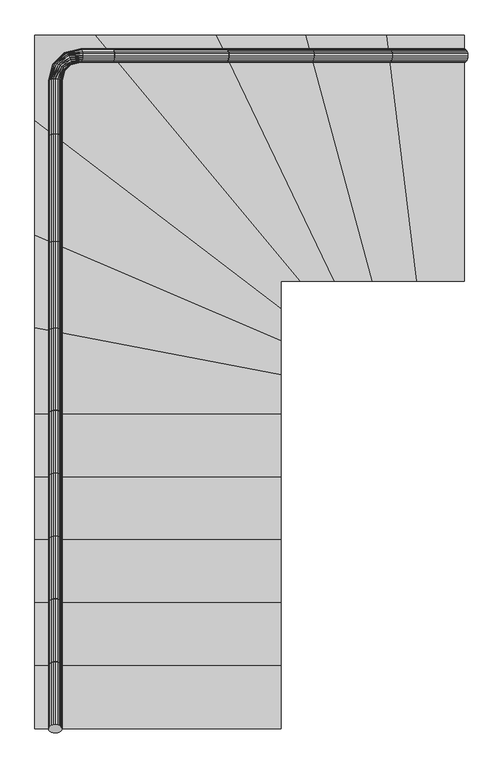
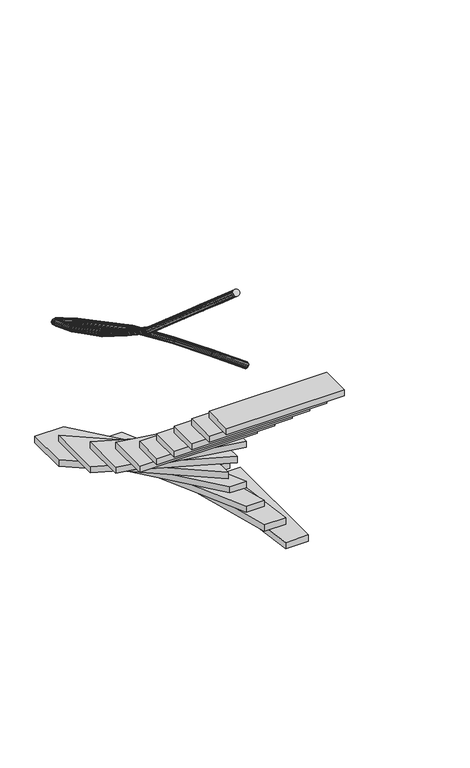
"""IFC4 building model written with IfcOpenShell, lengths in millimetres: stair geometry, 0_3d."""

from ifc_helpers import new_model, si_unit, frame, origin, origin_with_axes, place, context, project, spatial, polyline, outline, extrude, faceted_brep, source, transform, mapped, element, save


def stair_f0ca9b28(model_context):
    return source(origin(), model_context, "Body", "SolidModel", [
        extrude(outline(polyline([(1231.3290941, 1649.6053406), (1093.3486159, 1649.6053406), (662.4236343, 2549.6053406), (988.6709059, 2549.6053406), (1231.3290941, 1649.6053406)])), frame((0.0, 0.0, 400.0), z_axis=(0.0, 0.0, 1.0), x_axis=(1.0, 0.0, 0.0)), (0.0, 0.0, 1.0), 50.0),
        extrude(outline(polyline([(900.0, 705.003504), (900.0, 475.003504), (0.0, 475.003504), (0.0, 705.003504), (900.0, 705.003504)])), frame((0.0, 0.0, 2000.0), z_axis=(0.0, 0.0, 1.0), x_axis=(1.0, 0.0, 0.0)), (0.0, 0.0, 1.0), 50.0),
        extrude(outline(polyline([(1093.3486159, 1649.6053406), (970.0, 1649.6053406), (219.7566439, 2549.6053406), (662.4236343, 2549.6053406), (1093.3486159, 1649.6053406)])), frame((0.0, 0.0, 600.0), z_axis=(0.0, 0.0, 1.0), x_axis=(1.0, 0.0, 0.0)), (0.0, 0.0, 1.0), 50.0),
        extrude(outline(polyline([(1.2235871, -7.0656631), (0.0, 0.0), (1.2235871, 7.0656631), (4.7745751, 13.4396897), (10.3053687, 18.4981459), (17.2745751, 21.7458748), (25.0, 22.8649659), (32.7254249, 21.7458748), (39.6946313, 18.4981459), (45.2254249, 13.4396897), (48.7764129, 7.0656631), (50.0, 0.0), (48.7764129, -7.0656631), (45.2254249, -13.4396898), (39.6946313, -18.498146), (32.7254249, -21.7458748), (25.0, -22.864966), (17.2745751, -21.7458748), (10.3053687, -18.498146), (4.7745751, -13.4396898), (1.2235871, -7.0656631)])), frame((50.0, 475.003504, 3121.0), z_axis=(0.0, -0.7546055221635335, 0.6561787149247537), x_axis=(1.0, 0.0, 0.0)), (0.0, 0.0, 1.0), 304.7950131),
        extrude(outline(polyline([(1570.0, 1649.6053406), (1394.8371648, 1649.6053406), (1285.1628352, 2549.6053406), (1570.0, 2549.6053406), (1570.0, 1649.6053406)])), origin_with_axes(), (0.0, 0.0, 1.0), 50.0),
        extrude(outline(polyline([(1.2235871, -7.0656631), (0.0, 0.0), (1.2235871, 7.0656631), (4.7745751, 13.4396897), (10.3053687, 18.4981459), (17.2745751, 21.7458748), (25.0, 22.8649659), (32.7254249, 21.7458748), (39.6946313, 18.4981459), (45.2254249, 13.4396897), (48.7764129, 7.0656631), (50.0, 0.0), (48.7764129, -7.0656631), (45.2254249, -13.4396898), (39.6946313, -18.498146), (32.7254249, -21.7458748), (25.0, -22.864966), (17.2745751, -21.7458748), (10.3053687, -18.498146), (4.7745751, -13.4396898), (1.2235871, -7.0656631)])), frame((50.0, 935.003504, 2721.0), z_axis=(0.0, -0.7546055221635325, 0.6561787149247547), x_axis=(1.0, 0.0, 0.0)), (0.0, 0.0, 1.0), 304.7950131),
        faceted_brep([(51.2235871, 2175.7019192, 1914.5547212), (50.0, 2178.6155291, 1921.0), (51.2235871, 2181.5291389, 1927.4452788), (54.7745751, 2184.1575443, 1933.2596488), (60.3053687, 2186.2434586, 1937.8739589), (67.2745751, 2187.5826981, 1940.8365284), (75.0, 2188.0441685, 1941.8573603), (82.7254249, 2187.5826981, 1940.8365284), (89.6946313, 2186.2434586, 1937.8739589), (95.2254249, 2184.1575443, 1933.2596488), (98.7764129, 2181.5291389, 1927.4452788), (100.0, 2178.6155291, 1921.0), (98.7764129, 2175.7019192, 1914.5547212), (95.2254249, 2173.0735138, 1908.7403512), (89.6946313, 2170.9875995, 1904.1260411), (82.7254249, 2169.64836, 1901.1634716), (75.0, 2169.1868896, 1900.1426397), (67.2745751, 2169.64836, 1901.1634716), (60.3053687, 2170.9875995, 1904.1260411), (54.7745751, 2173.0735138, 1908.7403512), (51.2235871, 1789.2064798, 2127.1536239), (50.0, 1785.7199202, 2121.0), (51.2235871, 1782.2333607, 2114.8463761), (54.7745751, 1779.0880899, 2109.2951119), (60.3053687, 1776.5919889, 2104.8896036), (67.2745751, 1774.9893933, 2102.0610932), (75.0, 1774.4371766, 2101.0864549), (82.7254249, 1774.9893933, 2102.0610932), (89.6946313, 1776.5919889, 2104.8896036), (95.2254249, 1779.0880899, 2109.2951119), (98.7764129, 1782.2333607, 2114.8463761), (100.0, 1785.7199202, 2121.0), (98.7764129, 1789.2064798, 2127.1536239), (95.2254249, 1792.3517506, 2132.7048881), (89.6946313, 1794.8478516, 2137.1103964), (82.7254249, 1796.4504471, 2139.9389068), (75.0, 1797.0026639, 2140.9135451), (67.2745751, 1796.4504471, 2139.9389068), (60.3053687, 1794.8478516, 2137.1103964), (54.7745751, 1792.3517506, 2132.7048881)], [[[0, 1, 2, 3, 4, 5, 6, 7, 8, 9, 10, 11, 12, 13, 14, 15, 16, 17, 18, 19]], [[20, 21, 22, 23, 24, 25, 26, 27, 28, 29, 30, 31, 32, 33, 34, 35, 36, 37, 38, 39]], [[2, 1, 21, 20]], [[3, 2, 20, 39]], [[4, 3, 39, 38]], [[5, 4, 38, 37]], [[6, 5, 37, 36]], [[7, 6, 36, 35]], [[8, 7, 35, 34]], [[9, 8, 34, 33]], [[10, 9, 33, 32]], [[11, 10, 32, 31]], [[12, 11, 31, 30]], [[13, 12, 30, 29]], [[14, 13, 29, 28]], [[15, 14, 28, 27]], [[16, 15, 27, 26]], [[17, 16, 26, 25]], [[18, 17, 25, 24]], [[19, 18, 24, 23]], [[0, 19, 23, 22]], [[1, 0, 22, 21]]]),
        extrude(outline(polyline([(1.2235871, -7.0656631), (0.0, 0.0), (1.2235871, 7.0656631), (4.7745751, 13.4396897), (10.3053687, 18.4981459), (17.2745751, 21.7458748), (25.0, 22.8649659), (32.7254249, 21.7458748), (39.6946313, 18.4981459), (45.2254249, 13.4396897), (48.7764129, 7.0656631), (50.0, 0.0), (48.7764129, -7.0656631), (45.2254249, -13.4396898), (39.6946313, -18.498146), (32.7254249, -21.7458748), (25.0, -22.864966), (17.2745751, -21.7458748), (10.3053687, -18.498146), (4.7745751, -13.4396898), (1.2235871, -7.0656631)])), frame((50.0, 245.003504, 3321.0), z_axis=(0.0, -0.7546055221635316, 0.6561787149247558), x_axis=(1.0, 0.0, 0.0)), (0.0, 0.0, 1.0), 304.7950131),
        extrude(outline(polyline([(1.2235871, -7.0656631), (0.0, 0.0), (1.2235871, 7.0656631), (4.7745751, 13.4396897), (10.3053687, 18.4981459), (17.2745751, 21.7458748), (25.0, 22.8649659), (32.7254249, 21.7458748), (39.6946313, 18.4981459), (45.2254249, 13.4396897), (48.7764129, 7.0656631), (50.0, 0.0), (48.7764129, -7.0656631), (45.2254249, -13.4396898), (39.6946313, -18.498146), (32.7254249, -21.7458748), (25.0, -22.864966), (17.2745751, -21.7458748), (10.3053687, -18.498146), (4.7745751, -13.4396898), (1.2235871, -7.0656631)])), frame((50.0, 705.003504, 2921.0), z_axis=(0.0, -0.7546055221635325, 0.6561787149247547), x_axis=(1.0, 0.0, 0.0)), (0.0, 0.0, 1.0), 304.7950131),
        faceted_brep([(1004.9507123, 2498.3817535, 1315.1343723), (1008.8924216, 2499.6053406, 1321.0), (1012.8341309, 2498.3817535, 1326.8656277), (1016.3899982, 2494.8307654, 1332.1570869), (1019.2119505, 2489.2999719, 1336.3564127), (1021.0237554, 2482.3307654, 1339.0525459), (1021.6480608, 2474.6053406, 1339.98157), (1021.0237554, 2466.8799157, 1339.0525459), (1019.2119505, 2459.9107093, 1336.3564127), (1016.3899982, 2454.3799157, 1332.1570869), (1012.8341309, 2450.8289277, 1326.8656277), (1008.8924216, 2449.6053406, 1321.0), (1004.9507123, 2450.8289277, 1315.1343723), (1001.394845, 2454.3799157, 1309.8429131), (998.5728927, 2459.9107093, 1305.6435873), (996.7610878, 2466.8799157, 1302.9474541), (996.1367824, 2474.6053406, 1302.01843), (996.7610878, 2482.3307654, 1302.9474541), (998.5728927, 2489.2999719, 1305.6435873), (1001.394845, 2494.8307654, 1309.8429131), (701.7907267, 2498.3817535, 1527.177989), (698.3340494, 2499.6053406, 1521.0), (694.8773721, 2498.3817535, 1514.822011), (691.7590585, 2494.8307654, 1509.2487667), (689.2843508, 2489.2999719, 1504.8258149), (687.6954906, 2482.3307654, 1501.986105), (687.1480067, 2474.6053406, 1501.0076077), (687.6954906, 2466.8799157, 1501.986105), (689.2843508, 2459.9107093, 1504.8258149), (691.7590585, 2454.3799157, 1509.2487667), (694.8773721, 2450.8289277, 1514.822011), (698.3340494, 2449.6053406, 1521.0), (701.7907267, 2450.8289277, 1527.177989), (704.9090403, 2454.3799157, 1532.7512333), (707.383748, 2459.9107093, 1537.1741851), (708.9726082, 2466.8799157, 1540.013895), (709.5200921, 2474.6053406, 1540.9923923), (708.9726082, 2482.3307654, 1540.013895), (707.383748, 2489.2999719, 1537.1741851), (704.9090403, 2494.8307654, 1532.7512333)], [[[0, 1, 2, 3, 4, 5, 6, 7, 8, 9, 10, 11, 12, 13, 14, 15, 16, 17, 18, 19]], [[20, 21, 22, 23, 24, 25, 26, 27, 28, 29, 30, 31, 32, 33, 34, 35, 36, 37, 38, 39]], [[2, 1, 21, 20]], [[3, 2, 20, 39]], [[4, 3, 39, 38]], [[5, 4, 38, 37]], [[6, 5, 37, 36]], [[7, 6, 36, 35]], [[8, 7, 35, 34]], [[9, 8, 34, 33]], [[10, 9, 33, 32]], [[11, 10, 32, 31]], [[12, 11, 31, 30]], [[13, 12, 30, 29]], [[14, 13, 29, 28]], [[15, 14, 28, 27]], [[16, 15, 27, 26]], [[17, 16, 26, 25]], [[18, 17, 25, 24]], [[19, 18, 24, 23]], [[0, 19, 23, 22]], [[1, 0, 22, 21]]]),
        extrude(outline(polyline([(900.0, 1308.8458054), (900.0, 1165.003504), (0.0, 1165.003504), (0.0, 1481.1612025), (900.0, 1308.8458054)])), frame((0.0, 0.0, 1400.0), z_axis=(0.0, 0.0, 1.0), x_axis=(1.0, 0.0, 0.0)), (0.0, 0.0, 1.0), 50.0),
        faceted_brep([(51.2235871, 1462.9724676, 2315.0612017), (50.0, 1466.8015861, 2321.0), (51.2235871, 1470.6307046, 2326.9387983), (54.7745751, 1474.0850023, 2332.2962657), (60.3053687, 1476.8263485, 2336.5479759), (67.2745751, 1478.5864011, 2339.2777419), (75.0, 1479.1928739, 2340.2183552), (82.7254249, 1478.5864011, 2339.2777419), (89.6946313, 1476.8263485, 2336.5479759), (95.2254249, 1474.0850023, 2332.2962657), (98.7764129, 1470.6307046, 2326.9387983), (100.0, 1466.8015861, 2321.0), (98.7764129, 1462.9724676, 2315.0612017), (95.2254249, 1459.5181699, 2309.7037343), (89.6946313, 1456.7768237, 2305.4520241), (82.7254249, 1455.0167712, 2302.7222581), (75.0, 1454.4102984, 2301.7816448), (67.2745751, 1455.0167712, 2302.7222581), (60.3053687, 1456.7768237, 2305.4520241), (54.7745751, 1459.5181699, 2309.7037343), (51.2235871, 1169.2914591, 2526.6347297), (50.0, 1165.003504, 2521.0), (51.2235871, 1160.7155489, 2515.3652703), (54.7745751, 1156.8473287, 2510.2821071), (60.3053687, 1153.7774918, 2506.248086), (67.2745751, 1151.8065351, 2503.658085), (75.0, 1151.1273898, 2502.7656315), (82.7254249, 1151.8065351, 2503.658085), (89.6946313, 1153.7774918, 2506.248086), (95.2254249, 1156.8473287, 2510.2821071), (98.7764129, 1160.7155489, 2515.3652703), (100.0, 1165.003504, 2521.0), (98.7764129, 1169.2914591, 2526.6347297), (95.2254249, 1173.1596792, 2531.7178929), (89.6946313, 1176.2295162, 2535.751914), (82.7254249, 1178.2004728, 2538.341915), (75.0, 1178.8796182, 2539.2343685), (67.2745751, 1178.2004728, 2538.341915), (60.3053687, 1176.2295162, 2535.751914), (54.7745751, 1173.1596792, 2531.7178929)], [[[0, 1, 2, 3, 4, 5, 6, 7, 8, 9, 10, 11, 12, 13, 14, 15, 16, 17, 18, 19]], [[20, 21, 22, 23, 24, 25, 26, 27, 28, 29, 30, 31, 32, 33, 34, 35, 36, 37, 38, 39]], [[2, 1, 21, 20]], [[3, 2, 20, 39]], [[4, 3, 39, 38]], [[5, 4, 38, 37]], [[6, 5, 37, 36]], [[7, 6, 36, 35]], [[8, 7, 35, 34]], [[9, 8, 34, 33]], [[10, 9, 33, 32]], [[11, 10, 32, 31]], [[12, 11, 31, 30]], [[13, 12, 30, 29]], [[14, 13, 29, 28]], [[15, 14, 28, 27]], [[16, 15, 27, 26]], [[17, 16, 26, 25]], [[18, 17, 25, 24]], [[19, 18, 24, 23]], [[0, 19, 23, 22]], [[1, 0, 22, 21]]]),
        extrude(outline(polyline([(900.0, 245.003504), (900.0, 15.003504), (0.0, 15.003504), (0.0, 245.003504), (900.0, 245.003504)])), frame((0.0, 0.0, 2400.0), z_axis=(0.0, 0.0, 1.0), x_axis=(1.0, 0.0, 0.0)), (0.0, 0.0, 1.0), 50.0),
        faceted_brep([(1290.2002251, 2498.3817535, 1115.2467918), (1294.3023627, 2499.6053406, 1121.0), (1298.4045003, 2498.3817535, 1126.7532082), (1302.105092, 2494.8307654, 1131.9432522), (1305.0418983, 2489.2999719, 1136.0620945), (1306.927444, 2482.3307654, 1138.7065541), (1307.5771587, 2474.6053406, 1139.6177727), (1306.927444, 2466.8799157, 1138.7065541), (1305.0418983, 2459.9107093, 1136.0620945), (1302.105092, 2454.3799157, 1131.9432522), (1298.4045003, 2450.8289277, 1126.7532082), (1294.3023627, 2449.6053406, 1121.0), (1290.2002251, 2450.8289277, 1115.2467918), (1286.4996333, 2454.3799157, 1110.0567478), (1283.5628271, 2459.9107093, 1105.9379055), (1281.6772814, 2466.8799157, 1103.2934459), (1281.0275666, 2474.6053406, 1102.3822273), (1281.6772814, 2482.3307654, 1103.2934459), (1283.5628271, 2489.2999719, 1105.9379055), (1286.4996333, 2494.8307654, 1110.0567478), (1012.8341309, 2498.3817535, 1326.8656277), (1008.8924216, 2499.6053406, 1321.0), (1004.9507123, 2498.3817535, 1315.1343723), (1001.394845, 2494.8307654, 1309.8429131), (998.5728927, 2489.2999719, 1305.6435873), (996.7610878, 2482.3307654, 1302.9474541), (996.1367824, 2474.6053406, 1302.01843), (996.7610878, 2466.8799157, 1302.9474541), (998.5728927, 2459.9107093, 1305.6435873), (1001.394845, 2454.3799157, 1309.8429131), (1004.9507123, 2450.8289277, 1315.1343723), (1008.8924216, 2449.6053406, 1321.0), (1012.8341309, 2450.8289277, 1326.8656277), (1016.3899982, 2454.3799157, 1332.1570869), (1019.2119505, 2459.9107093, 1336.3564127), (1021.0237554, 2466.8799157, 1339.0525459), (1021.6480608, 2474.6053406, 1339.98157), (1021.0237554, 2482.3307654, 1339.0525459), (1019.2119505, 2489.2999719, 1336.3564127), (1016.3899982, 2494.8307654, 1332.1570869)], [[[0, 1, 2, 3, 4, 5, 6, 7, 8, 9, 10, 11, 12, 13, 14, 15, 16, 17, 18, 19]], [[20, 21, 22, 23, 24, 25, 26, 27, 28, 29, 30, 31, 32, 33, 34, 35, 36, 37, 38, 39]], [[2, 1, 21, 20]], [[3, 2, 20, 39]], [[4, 3, 39, 38]], [[5, 4, 38, 37]], [[6, 5, 37, 36]], [[7, 6, 36, 35]], [[8, 7, 35, 34]], [[9, 8, 34, 33]], [[10, 9, 33, 32]], [[11, 10, 32, 31]], [[12, 11, 31, 30]], [[13, 12, 30, 29]], [[14, 13, 29, 28]], [[15, 14, 28, 27]], [[16, 15, 27, 26]], [[17, 16, 26, 25]], [[18, 17, 25, 24]], [[19, 18, 24, 23]], [[0, 19, 23, 22]], [[1, 0, 22, 21]]]),
        extrude(outline(polyline([(970.0, 1649.6053406), (900.0, 1649.6053406), (900.0, 1549.6053406), (0.0, 2235.7982735), (0.0, 2549.6053406), (219.7566439, 2549.6053406), (970.0, 1649.6053406)])), frame((0.0, 0.0, 800.0), z_axis=(0.0, 0.0, 1.0), x_axis=(1.0, 0.0, 0.0)), (0.0, 0.0, 1.0), 50.0),
        faceted_brep([(279.4381704, 2498.3817535, 1714.5249729), (282.2769235, 2499.6053406, 1721.0), (285.1156767, 2498.3817535, 1727.4750271), (287.6765529, 2494.8307654, 1733.3162334), (289.7088757, 2489.2999719, 1737.951841), (291.0137073, 2482.3307654, 1740.9280843), (291.4633216, 2474.6053406, 1741.9536279), (291.0137073, 2466.8799157, 1740.9280843), (289.7088757, 2459.9107093, 1737.951841), (287.6765529, 2454.3799157, 1733.3162334), (285.1156767, 2450.8289277, 1727.4750271), (282.2769235, 2449.6053406, 1721.0), (279.4381704, 2450.8289277, 1714.5249729), (276.8772942, 2454.3799157, 1708.6837666), (274.8449714, 2459.9107093, 1704.048159), (273.5401398, 2466.8799157, 1701.0719157), (273.0905255, 2474.6053406, 1700.0463721), (273.5401398, 2482.3307654, 1701.0719157), (274.8449714, 2489.2999719, 1704.048159), (276.8772942, 2494.8307654, 1708.6837666), (51.2235871, 2181.5291389, 1927.4452788), (50.0, 2178.6155291, 1921.0), (51.2235871, 2175.7019192, 1914.5547212), (54.7745751, 2173.0735138, 1908.7403512), (60.3053687, 2170.9875995, 1904.1260411), (67.2745751, 2169.64836, 1901.1634716), (75.0, 2169.1868896, 1900.1426397), (82.7254249, 2169.64836, 1901.1634716), (89.6946313, 2170.9875995, 1904.1260411), (95.2254249, 2173.0735138, 1908.7403512), (98.7764129, 2175.7019192, 1914.5547212), (100.0, 2178.6155291, 1921.0), (98.7764129, 2181.5291389, 1927.4452788), (95.2254249, 2184.1575443, 1933.2596488), (89.6946313, 2186.2434586, 1937.8739589), (82.7254249, 2187.5826981, 1940.8365284), (75.0, 2188.0441685, 1941.8573603), (67.2745751, 2187.5826981, 1940.8365284), (60.3053687, 2186.2434586, 1937.8739589), (54.7745751, 2184.1575443, 1933.2596488), (167.9306386, 2499.6053406, 1766.4416225), (170.5400564, 2498.3817535, 1773.0077883), (172.8940462, 2494.8307654, 1778.931212), (174.762183, 2489.2999719, 1783.6320677), (175.9616007, 2482.3307654, 1786.6502029), (176.3748919, 2474.6053406, 1787.6901813), (175.9616007, 2466.8799157, 1786.6502029), (174.762183, 2459.9107093, 1783.6320677), (172.8940462, 2454.3799157, 1778.931212), (170.5400564, 2450.8289277, 1773.0077883), (167.9306386, 2449.6053406, 1766.4416225), (165.3212209, 2450.8289277, 1759.8754567), (162.9672311, 2454.3799157, 1753.9520329), (161.0990942, 2459.9107093, 1749.2511773), (159.8996765, 2466.8799157, 1746.2330421), (159.4863854, 2474.6053406, 1745.1930636), (159.8996765, 2482.3307654, 1746.2330421), (161.0990942, 2489.2999719, 1749.2511773), (162.9672311, 2494.8307654, 1753.9520329), (165.3212209, 2498.3817535, 1759.8754567), (106.9211768, 2484.8919306, 1790.5400059), (110.4511534, 2485.43029, 1796.7585422), (114.8111845, 2483.769642, 1802.3683648), (119.5744798, 2480.0725424, 1806.8203453), (124.2747747, 2474.7008892, 1809.6786927), (128.4519717, 2468.1804971, 1810.663612), (131.6971776, 2461.1496275, 1809.6786927), (133.692729, 2454.296511, 1806.8203453), (134.2432875, 2448.2919784, 1802.3683648), (133.2949605, 2443.723795, 1796.7585422), (130.940577, 2441.0391267, 1790.5400059), (127.4106003, 2440.5007673, 1784.3214696), (123.0505692, 2442.1614153, 1778.711647), (118.2872739, 2445.8585149, 1774.2596665), (113.586979, 2451.2301681, 1771.4013191), (109.409782, 2457.7505602, 1770.4163997), (106.1645761, 2464.7814298, 1771.4013191), (104.1690247, 2471.6345463, 1774.2596665), (103.6184662, 2477.639079, 1778.711647), (104.5667932, 2482.2072623, 1784.3214696), (64.7134099, 2442.6841638, 1816.2051752), (67.3980783, 2445.0385474, 1822.4237115), (71.9662616, 2445.9868743, 1828.0335341), (77.9707943, 2445.4363158, 1832.4855146), (84.8239108, 2443.4407644, 1835.343862), (91.8547803, 2440.1955585, 1836.3287814), (98.3751724, 2436.0183616, 1835.343862), (103.7468257, 2431.3180666, 1832.4855146), (107.4439253, 2426.5547714, 1828.0335341), (109.1045733, 2422.1947403, 1822.4237115), (108.5662139, 2418.6647636, 1816.2051752), (105.8815455, 2416.3103801, 1809.9866389), (101.3133622, 2415.3620531, 1804.3768163), (95.3088296, 2415.9126116, 1799.9248359), (88.4557131, 2417.908163, 1797.0664885), (81.4248435, 2421.1533689, 1796.0815691), (74.9044514, 2425.3305658, 1797.0664885), (69.5327981, 2430.0308608, 1799.9248359), (65.8356986, 2434.7941561, 1804.3768163), (64.1750506, 2439.1541871, 1809.9866389), (50.0, 2381.6747019, 1840.3035586), (51.2235871, 2384.2841197, 1846.8697244), (54.7745751, 2386.6381095, 1852.7931482), (60.3053687, 2388.5062463, 1857.4940039), (67.2745751, 2389.705664, 1860.512139), (75.0, 2390.1189552, 1861.5521175), (82.7254249, 2389.705664, 1860.512139), (89.6946313, 2388.5062463, 1857.4940039), (95.2254249, 2386.6381095, 1852.7931482), (98.7764129, 2384.2841197, 1846.8697244), (100.0, 2381.6747019, 1840.3035586), (98.7764129, 2379.0652842, 1833.7373928), (95.2254249, 2376.7112944, 1827.8139691), (89.6946313, 2374.8431575, 1823.1131134), (82.7254249, 2373.6437398, 1820.0949783), (75.0, 2373.2304487, 1819.0549998), (67.2745751, 2373.6437398, 1820.0949783), (60.3053687, 2374.8431575, 1823.1131134), (54.7745751, 2376.7112944, 1827.8139691), (51.2235871, 2379.0652842, 1833.7373928)], [[[0, 1, 2, 3, 4, 5, 6, 7, 8, 9, 10, 11, 12, 13, 14, 15, 16, 17, 18, 19]], [[20, 21, 22, 23, 24, 25, 26, 27, 28, 29, 30, 31, 32, 33, 34, 35, 36, 37, 38, 39]], [[2, 1, 40, 41]], [[3, 2, 41, 42]], [[4, 3, 42, 43]], [[5, 4, 43, 44]], [[6, 5, 44, 45]], [[7, 6, 45, 46]], [[8, 7, 46, 47]], [[9, 8, 47, 48]], [[10, 9, 48, 49]], [[11, 10, 49, 50]], [[12, 11, 50, 51]], [[13, 12, 51, 52]], [[14, 13, 52, 53]], [[15, 14, 53, 54]], [[16, 15, 54, 55]], [[17, 16, 55, 56]], [[18, 17, 56, 57]], [[19, 18, 57, 58]], [[0, 19, 58, 59]], [[1, 0, 59, 40]], [[41, 40, 60]], [[61, 41, 60]], [[42, 41, 61]], [[62, 42, 61]], [[43, 42, 62]], [[63, 43, 62]], [[44, 43, 63]], [[64, 44, 63]], [[45, 44, 64]], [[65, 45, 64]], [[46, 45, 65]], [[66, 46, 65]], [[47, 46, 66]], [[67, 47, 66]], [[48, 47, 67]], [[68, 48, 67]], [[49, 48, 68]], [[69, 49, 68]], [[50, 49, 69]], [[70, 50, 69]], [[51, 50, 70]], [[71, 51, 70]], [[52, 51, 71]], [[72, 52, 71]], [[53, 52, 72]], [[73, 53, 72]], [[54, 53, 73]], [[74, 54, 73]], [[55, 54, 74]], [[75, 55, 74]], [[56, 55, 75]], [[76, 56, 75]], [[57, 56, 76]], [[77, 57, 76]], [[58, 57, 77]], [[78, 58, 77]], [[59, 58, 78]], [[79, 59, 78]], [[40, 59, 79]], [[60, 40, 79]], [[61, 60, 80]], [[81, 61, 80]], [[62, 61, 81]], [[82, 62, 81]], [[63, 62, 82]], [[83, 63, 82]], [[64, 63, 83]], [[84, 64, 83]], [[65, 64, 84]], [[85, 65, 84]], [[66, 65, 85]], [[86, 66, 85]], [[67, 66, 86]], [[87, 67, 86]], [[68, 67, 87]], [[88, 68, 87]], [[69, 68, 88]], [[89, 69, 88]], [[70, 69, 89]], [[90, 70, 89]], [[71, 70, 90]], [[91, 71, 90]], [[72, 71, 91]], [[92, 72, 91]], [[73, 72, 92]], [[93, 73, 92]], [[74, 73, 93]], [[94, 74, 93]], [[75, 74, 94]], [[95, 75, 94]], [[76, 75, 95]], [[96, 76, 95]], [[77, 76, 96]], [[97, 77, 96]], [[78, 77, 97]], [[98, 78, 97]], [[79, 78, 98]], [[99, 79, 98]], [[60, 79, 99]], [[80, 60, 99]], [[81, 80, 100]], [[101, 81, 100]], [[82, 81, 101]], [[102, 82, 101]], [[83, 82, 102]], [[103, 83, 102]], [[84, 83, 103]], [[104, 84, 103]], [[85, 84, 104]], [[105, 85, 104]], [[86, 85, 105]], [[106, 86, 105]], [[87, 86, 106]], [[107, 87, 106]], [[88, 87, 107]], [[108, 88, 107]], [[89, 88, 108]], [[109, 89, 108]], [[90, 89, 109]], [[110, 90, 109]], [[91, 90, 110]], [[111, 91, 110]], [[92, 91, 111]], [[112, 92, 111]], [[93, 92, 112]], [[113, 93, 112]], [[94, 93, 113]], [[114, 94, 113]], [[95, 94, 114]], [[115, 95, 114]], [[96, 95, 115]], [[116, 96, 115]], [[97, 96, 116]], [[117, 97, 116]], [[98, 97, 117]], [[118, 98, 117]], [[99, 98, 118]], [[119, 99, 118]], [[80, 99, 119]], [[100, 80, 119]], [[101, 100, 21, 20]], [[102, 101, 20, 39]], [[103, 102, 39, 38]], [[104, 103, 38, 37]], [[105, 104, 37, 36]], [[106, 105, 36, 35]], [[107, 106, 35, 34]], [[108, 107, 34, 33]], [[109, 108, 33, 32]], [[110, 109, 32, 31]], [[111, 110, 31, 30]], [[112, 111, 30, 29]], [[113, 112, 29, 28]], [[114, 113, 28, 27]], [[115, 114, 27, 26]], [[116, 115, 26, 25]], [[117, 116, 25, 24]], [[118, 117, 24, 23]], [[119, 118, 23, 22]], [[100, 119, 22, 21]]]),
        extrude(outline(polyline([(900.0, 1165.003504), (900.0, 935.003504), (0.0, 935.003504), (0.0, 1165.003504), (900.0, 1165.003504)])), frame((0.0, 0.0, 1600.0), z_axis=(0.0, 0.0, 1.0), x_axis=(1.0, 0.0, 0.0)), (0.0, 0.0, 1.0), 50.0),
        extrude(outline(polyline([(1394.8371648, 1649.6053406), (1231.3290941, 1649.6053406), (988.6709059, 2549.6053406), (1285.1628352, 2549.6053406), (1394.8371648, 1649.6053406)])), frame((0.0, 0.0, 200.0), z_axis=(0.0, 0.0, 1.0), x_axis=(1.0, 0.0, 0.0)), (0.0, 0.0, 1.0), 50.0),
        extrude(outline(polyline([(900.0, 1432.7268587), (900.0, 1308.8458054), (0.0, 1481.1612025), (0.0, 1817.8101985), (900.0, 1432.7268587)])), frame((0.0, 0.0, 1200.0), z_axis=(0.0, 0.0, 1.0), x_axis=(1.0, 0.0, 0.0)), (0.0, 0.0, 1.0), 50.0),
        faceted_brep([(51.2235871, 1160.7155489, 2515.3652703), (50.0, 1165.003504, 2521.0), (51.2235871, 1169.2914591, 2526.6347297), (54.7745751, 1173.1596792, 2531.7178929), (60.3053687, 1176.2295162, 2535.751914), (67.2745751, 1178.2004728, 2538.341915), (75.0, 1178.8796182, 2539.2343685), (82.7254249, 1178.2004728, 2538.341915), (89.6946313, 1176.2295162, 2535.751914), (95.2254249, 1173.1596792, 2531.7178929), (98.7764129, 1169.2914591, 2526.6347297), (100.0, 1165.003504, 2521.0), (98.7764129, 1160.7155489, 2515.3652703), (95.2254249, 1156.8473287, 2510.2821071), (89.6946313, 1153.7774918, 2506.248086), (82.7254249, 1151.8065351, 2503.658085), (75.0, 1151.1273898, 2502.7656315), (67.2745751, 1151.8065351, 2503.658085), (60.3053687, 1153.7774918, 2506.248086), (54.7745751, 1156.8473287, 2510.2821071), (51.2235871, 939.6398417, 2726.3317884), (50.0, 935.003504, 2721.0), (51.2235871, 930.3671663, 2715.6682116), (54.7745751, 926.1846656, 2710.8583359), (60.3053687, 922.8654143, 2707.0411969), (67.2745751, 920.7343238, 2704.5904428), (75.0, 920.0, 2703.7459704), (82.7254249, 920.7343238, 2704.5904428), (89.6946313, 922.8654143, 2707.0411969), (95.2254249, 926.1846656, 2710.8583359), (98.7764129, 930.3671663, 2715.6682116), (100.0, 935.003504, 2721.0), (98.7764129, 939.6398417, 2726.3317884), (95.2254249, 943.8223423, 2731.1416641), (89.6946313, 947.1415936, 2734.9588031), (82.7254249, 949.2726842, 2737.4095572), (75.0, 950.0070079, 2738.2540296), (67.2745751, 949.2726842, 2737.4095572), (60.3053687, 947.1415936, 2734.9588031), (54.7745751, 943.8223423, 2731.1416641)], [[[0, 1, 2, 3, 4, 5, 6, 7, 8, 9, 10, 11, 12, 13, 14, 15, 16, 17, 18, 19]], [[20, 21, 22, 23, 24, 25, 26, 27, 28, 29, 30, 31, 32, 33, 34, 35, 36, 37, 38, 39]], [[2, 1, 21, 20]], [[3, 2, 20, 39]], [[4, 3, 39, 38]], [[5, 4, 38, 37]], [[6, 5, 37, 36]], [[7, 6, 36, 35]], [[8, 7, 35, 34]], [[9, 8, 34, 33]], [[10, 9, 33, 32]], [[11, 10, 32, 31]], [[12, 11, 31, 30]], [[13, 12, 30, 29]], [[14, 13, 29, 28]], [[15, 14, 28, 27]], [[16, 15, 27, 26]], [[17, 16, 26, 25]], [[18, 17, 25, 24]], [[19, 18, 24, 23]], [[0, 19, 23, 22]], [[1, 0, 22, 21]]]),
        faceted_brep([(694.8773721, 2498.3817535, 1514.822011), (698.3340494, 2499.6053406, 1521.0), (701.7907267, 2498.3817535, 1527.177989), (704.9090403, 2494.8307654, 1532.7512333), (707.383748, 2489.2999719, 1537.1741851), (708.9726082, 2482.3307654, 1540.013895), (709.5200921, 2474.6053406, 1540.9923923), (708.9726082, 2466.8799157, 1540.013895), (707.383748, 2459.9107093, 1537.1741851), (704.9090403, 2454.3799157, 1532.7512333), (701.7907267, 2450.8289277, 1527.177989), (698.3340494, 2449.6053406, 1521.0), (694.8773721, 2450.8289277, 1514.822011), (691.7590585, 2454.3799157, 1509.2487667), (689.2843508, 2459.9107093, 1504.8258149), (687.6954906, 2466.8799157, 1501.986105), (687.1480067, 2474.6053406, 1501.0076077), (687.6954906, 2482.3307654, 1501.986105), (689.2843508, 2489.2999719, 1504.8258149), (691.7590585, 2494.8307654, 1509.2487667), (285.1156767, 2498.3817535, 1727.4750271), (282.2769235, 2499.6053406, 1721.0), (279.4381704, 2498.3817535, 1714.5249729), (276.8772942, 2494.8307654, 1708.6837666), (274.8449714, 2489.2999719, 1704.048159), (273.5401398, 2482.3307654, 1701.0719157), (273.0905255, 2474.6053406, 1700.0463721), (273.5401398, 2466.8799157, 1701.0719157), (274.8449714, 2459.9107093, 1704.048159), (276.8772942, 2454.3799157, 1708.6837666), (279.4381704, 2450.8289277, 1714.5249729), (282.2769235, 2449.6053406, 1721.0), (285.1156767, 2450.8289277, 1727.4750271), (287.6765529, 2454.3799157, 1733.3162334), (289.7088757, 2459.9107093, 1737.951841), (291.0137073, 2466.8799157, 1740.9280843), (291.4633216, 2474.6053406, 1741.9536279), (291.0137073, 2482.3307654, 1740.9280843), (289.7088757, 2489.2999719, 1737.951841), (287.6765529, 2494.8307654, 1733.3162334)], [[[0, 1, 2, 3, 4, 5, 6, 7, 8, 9, 10, 11, 12, 13, 14, 15, 16, 17, 18, 19]], [[20, 21, 22, 23, 24, 25, 26, 27, 28, 29, 30, 31, 32, 33, 34, 35, 36, 37, 38, 39]], [[2, 1, 21, 20]], [[3, 2, 20, 39]], [[4, 3, 39, 38]], [[5, 4, 38, 37]], [[6, 5, 37, 36]], [[7, 6, 36, 35]], [[8, 7, 35, 34]], [[9, 8, 34, 33]], [[10, 9, 33, 32]], [[11, 10, 32, 31]], [[12, 11, 31, 30]], [[13, 12, 30, 29]], [[14, 13, 29, 28]], [[15, 14, 28, 27]], [[16, 15, 27, 26]], [[17, 16, 26, 25]], [[18, 17, 25, 24]], [[19, 18, 24, 23]], [[0, 19, 23, 22]], [[1, 0, 22, 21]]]),
        faceted_brep([(1565.8510641, 2498.3817535, 915.2807409), (1570.0, 2499.6053406, 921.0), (1574.1489359, 2498.3817535, 926.7192591), (1577.8917451, 2494.8307654, 931.8786773), (1580.8620552, 2489.2999719, 935.9732148), (1582.7691118, 2482.3307654, 938.6020697), (1583.4262386, 2474.6053406, 939.5079114), (1582.7691118, 2466.8799157, 938.6020697), (1580.8620552, 2459.9107093, 935.9732148), (1577.8917451, 2454.3799157, 931.8786773), (1574.1489359, 2450.8289277, 926.7192591), (1570.0, 2449.6053406, 921.0), (1565.8510641, 2450.8289277, 915.2807409), (1562.1082549, 2454.3799157, 910.1213227), (1559.1379448, 2459.9107093, 906.0267852), (1557.2308882, 2466.8799157, 903.3979303), (1556.5737614, 2474.6053406, 902.4920886), (1557.2308882, 2482.3307654, 903.3979303), (1559.1379448, 2489.2999719, 906.0267852), (1562.1082549, 2494.8307654, 910.1213227), (1298.4045003, 2498.3817535, 1126.7532082), (1294.3023627, 2499.6053406, 1121.0), (1290.2002251, 2498.3817535, 1115.2467918), (1286.4996333, 2494.8307654, 1110.0567478), (1283.5628271, 2489.2999719, 1105.9379055), (1281.6772814, 2482.3307654, 1103.2934459), (1281.0275666, 2474.6053406, 1102.3822273), (1281.6772814, 2466.8799157, 1103.2934459), (1283.5628271, 2459.9107093, 1105.9379055), (1286.4996333, 2454.3799157, 1110.0567478), (1290.2002251, 2450.8289277, 1115.2467918), (1294.3023627, 2449.6053406, 1121.0), (1298.4045003, 2450.8289277, 1126.7532082), (1302.105092, 2454.3799157, 1131.9432522), (1305.0418983, 2459.9107093, 1136.0620945), (1306.927444, 2466.8799157, 1138.7065541), (1307.5771587, 2474.6053406, 1139.6177727), (1306.927444, 2482.3307654, 1138.7065541), (1305.0418983, 2489.2999719, 1136.0620945), (1302.105092, 2494.8307654, 1131.9432522)], [[[0, 1, 2, 3, 4, 5, 6, 7, 8, 9, 10, 11, 12, 13, 14, 15, 16, 17, 18, 19]], [[20, 21, 22, 23, 24, 25, 26, 27, 28, 29, 30, 31, 32, 33, 34, 35, 36, 37, 38, 39]], [[2, 1, 21, 20]], [[3, 2, 20, 39]], [[4, 3, 39, 38]], [[5, 4, 38, 37]], [[6, 5, 37, 36]], [[7, 6, 36, 35]], [[8, 7, 35, 34]], [[9, 8, 34, 33]], [[10, 9, 33, 32]], [[11, 10, 32, 31]], [[12, 11, 31, 30]], [[13, 12, 30, 29]], [[14, 13, 29, 28]], [[15, 14, 28, 27]], [[16, 15, 27, 26]], [[17, 16, 26, 25]], [[18, 17, 25, 24]], [[19, 18, 24, 23]], [[0, 19, 23, 22]], [[1, 0, 22, 21]]]),
        extrude(outline(polyline([(900.0, 935.003504), (900.0, 705.003504), (0.0, 705.003504), (0.0, 935.003504), (900.0, 935.003504)])), frame((0.0, 0.0, 1800.0), z_axis=(0.0, 0.0, 1.0), x_axis=(1.0, 0.0, 0.0)), (0.0, 0.0, 1.0), 50.0),
        extrude(outline(polyline([(900.0, 475.003504), (900.0, 245.003504), (0.0, 245.003504), (0.0, 475.003504), (900.0, 475.003504)])), frame((0.0, 0.0, 2200.0), z_axis=(0.0, 0.0, 1.0), x_axis=(1.0, 0.0, 0.0)), (0.0, 0.0, 1.0), 50.0),
        extrude(outline(polyline([(900.0, 1549.6053406), (900.0, 1432.7268587), (0.0, 1817.8101985), (0.0, 2235.7982735), (900.0, 1549.6053406)])), frame((0.0, 0.0, 1000.0), z_axis=(0.0, 0.0, 1.0), x_axis=(1.0, 0.0, 0.0)), (0.0, 0.0, 1.0), 50.0),
        faceted_brep([(51.2235871, 1782.2333607, 2114.8463761), (50.0, 1785.7199202, 2121.0), (51.2235871, 1789.2064798, 2127.1536239), (54.7745751, 1792.3517506, 2132.7048881), (60.3053687, 1794.8478516, 2137.1103964), (67.2745751, 1796.4504471, 2139.9389068), (75.0, 1797.0026639, 2140.9135451), (82.7254249, 1796.4504471, 2139.9389068), (89.6946313, 1794.8478516, 2137.1103964), (95.2254249, 1792.3517506, 2132.7048881), (98.7764129, 1789.2064798, 2127.1536239), (100.0, 1785.7199202, 2121.0), (98.7764129, 1782.2333607, 2114.8463761), (95.2254249, 1779.0880899, 2109.2951119), (89.6946313, 1776.5919889, 2104.8896036), (82.7254249, 1774.9893933, 2102.0610932), (75.0, 1774.4371766, 2101.0864549), (67.2745751, 1774.9893933, 2102.0610932), (60.3053687, 1776.5919889, 2104.8896036), (54.7745751, 1779.0880899, 2109.2951119), (51.2235871, 1470.6307046, 2326.9387983), (50.0, 1466.8015861, 2321.0), (51.2235871, 1462.9724676, 2315.0612017), (54.7745751, 1459.5181699, 2309.7037343), (60.3053687, 1456.7768237, 2305.4520241), (67.2745751, 1455.0167712, 2302.7222581), (75.0, 1454.4102984, 2301.7816448), (82.7254249, 1455.0167712, 2302.7222581), (89.6946313, 1456.7768237, 2305.4520241), (95.2254249, 1459.5181699, 2309.7037343), (98.7764129, 1462.9724676, 2315.0612017), (100.0, 1466.8015861, 2321.0), (98.7764129, 1470.6307046, 2326.9387983), (95.2254249, 1474.0850023, 2332.2962657), (89.6946313, 1476.8263485, 2336.5479759), (82.7254249, 1478.5864011, 2339.2777419), (75.0, 1479.1928739, 2340.2183552), (67.2745751, 1478.5864011, 2339.2777419), (60.3053687, 1476.8263485, 2336.5479759), (54.7745751, 1474.0850023, 2332.2962657)], [[[0, 1, 2, 3, 4, 5, 6, 7, 8, 9, 10, 11, 12, 13, 14, 15, 16, 17, 18, 19]], [[20, 21, 22, 23, 24, 25, 26, 27, 28, 29, 30, 31, 32, 33, 34, 35, 36, 37, 38, 39]], [[2, 1, 21, 20]], [[3, 2, 20, 39]], [[4, 3, 39, 38]], [[5, 4, 38, 37]], [[6, 5, 37, 36]], [[7, 6, 36, 35]], [[8, 7, 35, 34]], [[9, 8, 34, 33]], [[10, 9, 33, 32]], [[11, 10, 32, 31]], [[12, 11, 31, 30]], [[13, 12, 30, 29]], [[14, 13, 29, 28]], [[15, 14, 28, 27]], [[16, 15, 27, 26]], [[17, 16, 26, 25]], [[18, 17, 25, 24]], [[19, 18, 24, 23]], [[0, 19, 23, 22]], [[1, 0, 22, 21]]]),
    ])


if __name__ == "__main__":
    model = new_model("IFC4")
    model_context = context("Model", 3, world=origin())
    ifc_project = project(units=[si_unit("LENGTHUNIT", "METRE", prefix="MILLI")], contexts=[model_context])
    site = spatial("IfcSite", under=ifc_project)
    building = spatial("IfcBuilding", under=site)
    placement = place(None, origin())
    stair_shape = stair_f0ca9b28(model_context)
    element("IfcStair", 1, ObjectType="0_3d", at=placement, inside=building, context=model_context, shape_type="MappedRepresentation", body=[
        mapped(stair_shape, transform((0.0, 0.0, 0.0), x_axis=(1.0, 0.0, 0.0), y_axis=(0.0, 1.0, 0.0), z_axis=(0.0, 0.0, 1.0))),
    ])
    save(model, "model.ifc")

# Revit data of these elements
# Element 1 (IfcStair, "0_3d")
#   Materials on its faces: "*1", "weiss"
# Materials
#   "*1": class "Unassigned", colour RGB 175 175 175, transparency 0
#   "weiss": class "Unassigned", colour RGB 255 255 255, transparency 0
